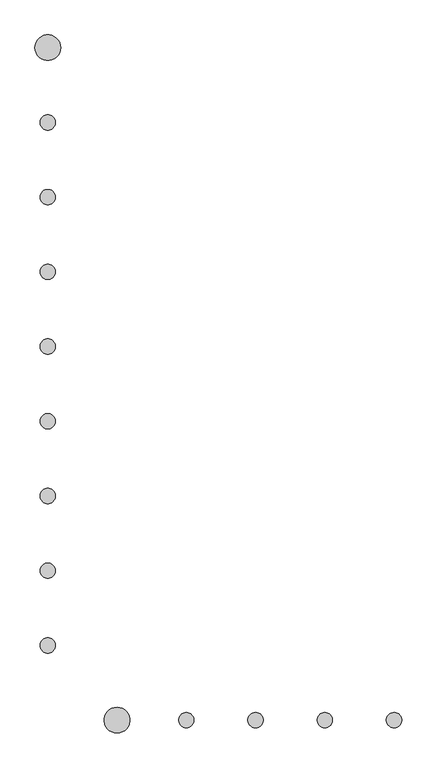
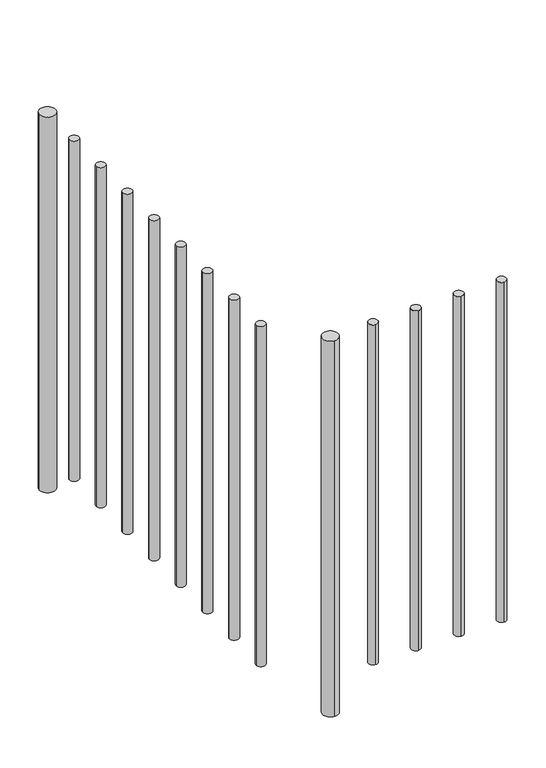
"""IFC4 building model written with IfcOpenShell, lengths in millimetres: railing geometry."""

import ifcopenshell
import ifcopenshell.guid

model = None  # the IFC model being written
_history = None  # IfcOwnerHistory: only IFC2X3 demands one
_inside = {}  # id of a spatial element -> (the spatial element, [elements in it])
_under = {}  # id of a project, library or spatial element -> (it, [spatial elements below it])
_declared = {}  # id of a project -> (the project, [libraries it declares])
_typed = {}  # id of a type object -> (the type object, [elements of that type])
_made_of = {}  # id of a material, layer set ... -> (it, [elements and type objects made of it])


def new_model(schema):
    """Start an empty IFC model of exactly this schema.

    Asked for "IFC4X3", IfcOpenShell would pick the latest addendum, in which some entities
    have other attributes; the version numbers below select the first issue.
    IFC2X3 requires an IfcOwnerHistory on every rooted entity: one is made here for all.
    """
    global model, _history
    if schema == "IFC4X3":
        model = ifcopenshell.file(schema_version=(4, 3, 0, 0))
    else:
        model = ifcopenshell.file(schema=schema)
    _inside.clear()
    _under.clear()
    _declared.clear()
    _typed.clear()
    _made_of.clear()
    _history = None
    if model.schema == "IFC2X3":
        org = make("IfcOrganization", Name="unknown")
        user = make(
            "IfcPersonAndOrganization",
            ThePerson=make("IfcPerson", FamilyName="unknown"),
            TheOrganization=org,
        )
        app = make(
            "IfcApplication",
            ApplicationDeveloper=org,
            Version="unknown",
            ApplicationFullName="unknown",
            ApplicationIdentifier="unknown",
        )
        _history = make(
            "IfcOwnerHistory",
            OwningUser=user,
            OwningApplication=app,
            ChangeAction="ADDED",
            CreationDate=0,
        )
    return model


def make(cls, **values):
    """One entity of the class cls with the attributes given. An attribute that is None is left unset."""
    return model.create_entity(
        cls, **{name: value for name, value in values.items() if value is not None}
    )


def rooted(cls, **values):
    """An entity with a GlobalId (a new one), such as an element, a storey or a relation."""
    return make(cls, GlobalId=ifcopenshell.guid.new(), OwnerHistory=_history, **values)


def si_unit(unit_type, name, prefix=None):
    """IfcSIUnit, for example si_unit("LENGTHUNIT", "METRE", prefix="MILLI")."""
    return make("IfcSIUnit", UnitType=unit_type, Prefix=prefix, Name=name)


def assignment(units):
    """IfcUnitAssignment: the units of a project."""
    return None if units is None else make("IfcUnitAssignment", Units=units)


def point(xyz):
    """IfcCartesianPoint."""
    return None if xyz is None else make("IfcCartesianPoint", Coordinates=xyz)


def direction(xyz):
    """IfcDirection."""
    return None if xyz is None else make("IfcDirection", DirectionRatios=xyz)


def frame(location, z_axis=None, x_axis=None):
    """IfcAxis2Placement3D, a coordinate frame: its origin and axes. An axis left out is left unset."""
    return make(
        "IfcAxis2Placement3D",
        Location=point(location),
        Axis=direction(z_axis),
        RefDirection=direction(x_axis),
    )


def frame_2d(location, x_axis=None):
    """IfcAxis2Placement2D, a coordinate frame in the plane: its origin and x axis."""
    return make(
        "IfcAxis2Placement2D", Location=point(location), RefDirection=direction(x_axis)
    )


def origin():
    """The frame at (0, 0, 0) with its axes left unset."""
    return frame((0.0, 0.0, 0.0))


def place(relative_to, where):
    """IfcLocalPlacement: puts the frame where relative to a parent placement (None: the world)."""
    return make(
        "IfcLocalPlacement", PlacementRelTo=relative_to, RelativePlacement=where
    )


def context(
    kind, dimensions, precision=None, world=None, true_north=None, identifier=None
):
    """IfcGeometricRepresentationContext, for example the 3D "Model" context."""
    return make(
        "IfcGeometricRepresentationContext",
        ContextIdentifier=identifier,
        ContextType=kind,
        CoordinateSpaceDimension=dimensions,
        Precision=precision,
        WorldCoordinateSystem=world,
        TrueNorth=true_north,
    )


def project(units=None, contexts=None):
    """IfcProject with its units and contexts."""
    return rooted(
        "IfcProject",
        Name="project",
        RepresentationContexts=contexts,
        UnitsInContext=assignment(units),
    )


def spatial(cls, under=None, at=None, **own):
    """A site, building, storey or space (cls), placed at a placement, below another one or the project."""
    s = rooted(cls, ObjectPlacement=at, **own)
    if under is not None:
        _under.setdefault(under.id(), (under, []))[1].append(s)
    return s


def circle_curve(where, radius):
    """IfcCircle in the frame where."""
    return make("IfcCircle", Position=where, Radius=radius)


def trimmed(basis, trim1, trim2, sense, master):
    """IfcTrimmedCurve: the piece of a basis curve between two trims."""
    return make(
        "IfcTrimmedCurve",
        BasisCurve=basis,
        Trim1=trim1,
        Trim2=trim2,
        SenseAgreement=sense,
        MasterRepresentation=master,
    )


def segment(curve, same_sense, transition):
    """IfcCompositeCurveSegment."""
    return make(
        "IfcCompositeCurveSegment",
        Transition=transition,
        SameSense=same_sense,
        ParentCurve=curve,
    )


def composite_curve(segments, self_intersect=None):
    """IfcCompositeCurve: segments joined end to end."""
    return make("IfcCompositeCurve", Segments=segments, SelfIntersect=self_intersect)


def outline(outer, holes=None, kind="AREA"):
    """IfcArbitraryClosedProfileDef: a profile drawn as a closed curve; with holes, ...WithVoids."""
    if holes is None:
        return make("IfcArbitraryClosedProfileDef", ProfileType=kind, OuterCurve=outer)
    return make(
        "IfcArbitraryProfileDefWithVoids",
        ProfileType=kind,
        OuterCurve=outer,
        InnerCurves=holes,
    )


def extrude(swept, where, along, depth):
    """IfcExtrudedAreaSolid: the profile swept, set in the frame where, extruded along a direction by depth."""
    return make(
        "IfcExtrudedAreaSolid",
        SweptArea=swept,
        Position=where,
        ExtrudedDirection=direction(along),
        Depth=depth,
    )


def shape(context_of_items, identifier, shape_type, items):
    """IfcShapeRepresentation: the items that make up one representation, for example the "Body"."""
    return make(
        "IfcShapeRepresentation",
        ContextOfItems=context_of_items,
        RepresentationIdentifier=identifier,
        RepresentationType=shape_type,
        Items=items,
    )


def source(mapping_origin, context_of_items, identifier, shape_type, items):
    """IfcRepresentationMap: a shape defined once, which mapped items show again and again."""
    return make(
        "IfcRepresentationMap",
        MappingOrigin=mapping_origin,
        MappedRepresentation=shape(context_of_items, identifier, shape_type, items),
    )


def transform(
    local_origin,
    x_axis=None,
    y_axis=None,
    z_axis=None,
    scale=None,
    scale2=None,
    scale3=None,
    uniform=True,
):
    """IfcCartesianTransformationOperator3D, or its non-uniform kind. x_axis, y_axis, z_axis: its Axis1, 2, 3."""
    if uniform:
        return make(
            "IfcCartesianTransformationOperator3D",
            Axis1=direction(x_axis),
            Axis2=direction(y_axis),
            LocalOrigin=point(local_origin),
            Scale=scale,
            Axis3=direction(z_axis),
        )
    return make(
        "IfcCartesianTransformationOperator3DnonUniform",
        Axis1=direction(x_axis),
        Axis2=direction(y_axis),
        LocalOrigin=point(local_origin),
        Scale=scale,
        Axis3=direction(z_axis),
        Scale2=scale2,
        Scale3=scale3,
    )


def mapped(mapping_source, mapping_target):
    """IfcMappedItem: shows the shape of a source again, moved by a transform."""
    return make(
        "IfcMappedItem", MappingSource=mapping_source, MappingTarget=mapping_target
    )


def made_of(thing, what):
    """Note that an element or type object is made of a material, layer set ...; save() writes the relation."""
    if what is not None:
        _made_of.setdefault(what.id(), (what, []))[1].append(thing)
    return thing


def element(
    cls,
    number,
    at=None,
    inside=None,
    cuts=None,
    type_object=None,
    material=None,
    context=None,
    identifier="Body",
    shape_type=None,
    held_by="IfcProductDefinitionShape",
    body=None,
    shapes=None,
    **own,
):
    """One element of the class cls, such as IfcWall. Its Tag is "e" and its number.

    at: its placement. inside: the storey or other place that contains it. cuts: it is an
    opening in that element (IfcRelVoidsElement). A single representation is given by context,
    identifier, shape_type and body (its items); several are given by shapes. held_by: the class
    of the entity that holds the representations. save() writes the other relations.
    """
    e = rooted(cls, Tag="e%d" % number, ObjectPlacement=at, **own)
    if body is not None:
        shapes = [shape(context, identifier, shape_type, body)]
    if shapes is not None:
        e.Representation = make(held_by, Representations=shapes)
    if inside is not None:
        _inside.setdefault(inside.id(), (inside, []))[1].append(e)
    if cuts is not None:
        rooted(
            "IfcRelVoidsElement", RelatingBuildingElement=cuts, RelatedOpeningElement=e
        )
    if type_object is not None:
        _typed.setdefault(type_object.id(), (type_object, []))[1].append(e)
    return made_of(e, material)


def aggregate(whole, parts):
    """IfcRelAggregates: a whole, such as a stair, and the parts it consists of."""
    return rooted("IfcRelAggregates", RelatingObject=whole, RelatedObjects=parts)


def save(model, path):
    """Write the relations noted so far, then the file.

    IfcRelAggregates (storeys below a building ...), IfcRelContainedInSpatialStructure (elements
    in a storey), IfcRelDefinesByType, IfcRelAssociatesMaterial and IfcRelDeclares: one each for
    every whole, place, type object, material and project.
    """
    for whole, parts in _under.values():
        aggregate(whole, parts)
    for where, things in _inside.values():
        rooted(
            "IfcRelContainedInSpatialStructure",
            RelatedElements=things,
            RelatingStructure=where,
        )
    for kind, things in _typed.values():
        rooted("IfcRelDefinesByType", RelatedObjects=things, RelatingType=kind)
    for what, things in _made_of.values():
        rooted("IfcRelAssociatesMaterial", RelatedObjects=things, RelatingMaterial=what)
    for by, libraries in _declared.values():
        rooted("IfcRelDeclares", RelatingContext=by, RelatedDefinitions=libraries)
    model.write(path)


def railing_35eac12f(model_context):
    return source(origin(), model_context, "Body", "SweptSolid", [
        extrude(outline(composite_curve([segment(trimmed(circle_curve(frame_2d((-2709.174449, -8163.7965465)), 12.5), [point((-2709.174449, -8176.2965465))], [point((-2709.174449, -8151.2965465))], False, "CARTESIAN"), True, "CONTINUOUS"), segment(trimmed(circle_curve(frame_2d((-2709.174449, -8163.7965465)), 12.5), [point((-2709.174449, -8151.2965465))], [point((-2709.174449, -8176.2965465))], False, "CARTESIAN"), True, "CONTINUOUS")], self_intersect=False)), frame((0.0, 0.0, 3500.0), z_axis=(0.0, 0.0, 1.0), x_axis=(1.0, 0.0, 0.0)), (0.0, 0.0, 1.0), 949.2),
        extrude(outline(composite_curve([segment(trimmed(circle_curve(frame_2d((-2822.314449, -8163.7965465)), 12.5), [point((-2822.314449, -8176.2965465))], [point((-2822.314449, -8151.2965465))], False, "CARTESIAN"), True, "CONTINUOUS"), segment(trimmed(circle_curve(frame_2d((-2822.314449, -8163.7965465)), 12.5), [point((-2822.314449, -8151.2965465))], [point((-2822.314449, -8176.2965465))], False, "CARTESIAN"), True, "CONTINUOUS")], self_intersect=False)), frame((0.0, 0.0, 3500.0), z_axis=(0.0, 0.0, 1.0), x_axis=(1.0, 0.0, 0.0)), (0.0, 0.0, 1.0), 949.2),
        extrude(outline(composite_curve([segment(trimmed(circle_curve(frame_2d((-2935.454449, -8163.7965465)), 12.5), [point((-2935.454449, -8176.2965465))], [point((-2935.454449, -8151.2965465))], False, "CARTESIAN"), True, "CONTINUOUS"), segment(trimmed(circle_curve(frame_2d((-2935.454449, -8163.7965465)), 12.5), [point((-2935.454449, -8151.2965465))], [point((-2935.454449, -8176.2965465))], False, "CARTESIAN"), True, "CONTINUOUS")], self_intersect=False)), frame((0.0, 0.0, 3500.0), z_axis=(0.0, 0.0, 1.0), x_axis=(1.0, 0.0, 0.0)), (0.0, 0.0, 1.0), 949.2),
        extrude(outline(composite_curve([segment(trimmed(circle_curve(frame_2d((-3048.594449, -8163.7965465)), 12.5), [point((-3048.594449, -8176.2965465))], [point((-3048.594449, -8151.2965465))], False, "CARTESIAN"), True, "CONTINUOUS"), segment(trimmed(circle_curve(frame_2d((-3048.594449, -8163.7965465)), 12.5), [point((-3048.594449, -8151.2965465))], [point((-3048.594449, -8176.2965465))], False, "CARTESIAN"), True, "CONTINUOUS")], self_intersect=False)), frame((0.0, 0.0, 3500.0), z_axis=(0.0, 0.0, 1.0), x_axis=(1.0, 0.0, 0.0)), (0.0, 0.0, 1.0), 949.2),
        extrude(outline(composite_curve([segment(trimmed(circle_curve(frame_2d((-3161.734449, -8163.7965465)), 21.0), [point((-3161.734449, -8184.7965465))], [point((-3161.734449, -8142.7965465))], False, "CARTESIAN"), True, "CONTINUOUS"), segment(trimmed(circle_curve(frame_2d((-3161.734449, -8163.7965465)), 21.0), [point((-3161.734449, -8142.7965465))], [point((-3161.734449, -8184.7965465))], False, "CARTESIAN"), True, "CONTINUOUS")], self_intersect=False)), frame((0.0, 0.0, 3400.0), z_axis=(0.0, 0.0, 1.0), x_axis=(1.0, 0.0, 0.0)), (0.0, 0.0, 1.0), 1049.2),
        extrude(outline(composite_curve([segment(trimmed(circle_curve(frame_2d((-3274.874449, -8041.7565465)), 12.5), [point((-3287.374449, -8041.7565465))], [point((-3262.374449, -8041.7565465))], False, "CARTESIAN"), True, "CONTINUOUS"), segment(trimmed(circle_curve(frame_2d((-3274.874449, -8041.7565465)), 12.5), [point((-3262.374449, -8041.7565465))], [point((-3287.374449, -8041.7565465))], False, "CARTESIAN"), True, "CONTINUOUS")], self_intersect=False)), frame((0.0, 0.0, 3500.0), z_axis=(0.0, 0.0, 1.0), x_axis=(1.0, 0.0, 0.0)), (0.0, 0.0, 1.0), 949.2),
        extrude(outline(composite_curve([segment(trimmed(circle_curve(frame_2d((-3274.874449, -7919.7165465)), 12.5), [point((-3287.374449, -7919.7165465))], [point((-3262.374449, -7919.7165465))], False, "CARTESIAN"), True, "CONTINUOUS"), segment(trimmed(circle_curve(frame_2d((-3274.874449, -7919.7165465)), 12.5), [point((-3262.374449, -7919.7165465))], [point((-3287.374449, -7919.7165465))], False, "CARTESIAN"), True, "CONTINUOUS")], self_intersect=False)), frame((0.0, 0.0, 3500.0), z_axis=(0.0, 0.0, 1.0), x_axis=(1.0, 0.0, 0.0)), (0.0, 0.0, 1.0), 949.2),
        extrude(outline(composite_curve([segment(trimmed(circle_curve(frame_2d((-3274.874449, -7797.6765465)), 12.5), [point((-3287.374449, -7797.6765465))], [point((-3262.374449, -7797.6765465))], False, "CARTESIAN"), True, "CONTINUOUS"), segment(trimmed(circle_curve(frame_2d((-3274.874449, -7797.6765465)), 12.5), [point((-3262.374449, -7797.6765465))], [point((-3287.374449, -7797.6765465))], False, "CARTESIAN"), True, "CONTINUOUS")], self_intersect=False)), frame((0.0, 0.0, 3500.0), z_axis=(0.0, 0.0, 1.0), x_axis=(1.0, 0.0, 0.0)), (0.0, 0.0, 1.0), 949.2),
        extrude(outline(composite_curve([segment(trimmed(circle_curve(frame_2d((-3274.874449, -7675.6365465)), 12.5), [point((-3287.374449, -7675.6365465))], [point((-3262.374449, -7675.6365465))], False, "CARTESIAN"), True, "CONTINUOUS"), segment(trimmed(circle_curve(frame_2d((-3274.874449, -7675.6365465)), 12.5), [point((-3262.374449, -7675.6365465))], [point((-3287.374449, -7675.6365465))], False, "CARTESIAN"), True, "CONTINUOUS")], self_intersect=False)), frame((0.0, 0.0, 3500.0), z_axis=(0.0, 0.0, 1.0), x_axis=(1.0, 0.0, 0.0)), (0.0, 0.0, 1.0), 949.2),
        extrude(outline(composite_curve([segment(trimmed(circle_curve(frame_2d((-3274.874449, -7553.5965465)), 12.5), [point((-3287.374449, -7553.5965465))], [point((-3262.374449, -7553.5965465))], False, "CARTESIAN"), True, "CONTINUOUS"), segment(trimmed(circle_curve(frame_2d((-3274.874449, -7553.5965465)), 12.5), [point((-3262.374449, -7553.5965465))], [point((-3287.374449, -7553.5965465))], False, "CARTESIAN"), True, "CONTINUOUS")], self_intersect=False)), frame((0.0, 0.0, 3500.0), z_axis=(0.0, 0.0, 1.0), x_axis=(1.0, 0.0, 0.0)), (0.0, 0.0, 1.0), 949.2),
        extrude(outline(composite_curve([segment(trimmed(circle_curve(frame_2d((-3274.874449, -7431.5565465)), 12.5), [point((-3287.374449, -7431.5565465))], [point((-3262.374449, -7431.5565465))], False, "CARTESIAN"), True, "CONTINUOUS"), segment(trimmed(circle_curve(frame_2d((-3274.874449, -7431.5565465)), 12.5), [point((-3262.374449, -7431.5565465))], [point((-3287.374449, -7431.5565465))], False, "CARTESIAN"), True, "CONTINUOUS")], self_intersect=False)), frame((0.0, 0.0, 3500.0), z_axis=(0.0, 0.0, 1.0), x_axis=(1.0, 0.0, 0.0)), (0.0, 0.0, 1.0), 949.2),
        extrude(outline(composite_curve([segment(trimmed(circle_curve(frame_2d((-3274.874449, -7309.5165465)), 12.5), [point((-3287.374449, -7309.5165465))], [point((-3262.374449, -7309.5165465))], False, "CARTESIAN"), True, "CONTINUOUS"), segment(trimmed(circle_curve(frame_2d((-3274.874449, -7309.5165465)), 12.5), [point((-3262.374449, -7309.5165465))], [point((-3287.374449, -7309.5165465))], False, "CARTESIAN"), True, "CONTINUOUS")], self_intersect=False)), frame((0.0, 0.0, 3500.0), z_axis=(0.0, 0.0, 1.0), x_axis=(1.0, 0.0, 0.0)), (0.0, 0.0, 1.0), 949.2),
        extrude(outline(composite_curve([segment(trimmed(circle_curve(frame_2d((-3274.874449, -7187.4765465)), 12.5), [point((-3287.374449, -7187.4765465))], [point((-3262.374449, -7187.4765465))], False, "CARTESIAN"), True, "CONTINUOUS"), segment(trimmed(circle_curve(frame_2d((-3274.874449, -7187.4765465)), 12.5), [point((-3262.374449, -7187.4765465))], [point((-3287.374449, -7187.4765465))], False, "CARTESIAN"), True, "CONTINUOUS")], self_intersect=False)), frame((0.0, 0.0, 3500.0), z_axis=(0.0, 0.0, 1.0), x_axis=(1.0, 0.0, 0.0)), (0.0, 0.0, 1.0), 949.2),
        extrude(outline(composite_curve([segment(trimmed(circle_curve(frame_2d((-3274.874449, -7065.4365465)), 21.0), [point((-3295.874449, -7065.4365465))], [point((-3253.874449, -7065.4365465))], False, "CARTESIAN"), True, "CONTINUOUS"), segment(trimmed(circle_curve(frame_2d((-3274.874449, -7065.4365465)), 21.0), [point((-3253.874449, -7065.4365465))], [point((-3295.874449, -7065.4365465))], False, "CARTESIAN"), True, "CONTINUOUS")], self_intersect=False)), frame((0.0, 0.0, 3400.0), z_axis=(0.0, 0.0, 1.0), x_axis=(1.0, 0.0, 0.0)), (0.0, 0.0, 1.0), 1049.2),
    ])


if __name__ == "__main__":
    model = new_model("IFC4")
    model_context = context("Model", 3, world=origin())
    ifc_project = project(units=[si_unit("LENGTHUNIT", "METRE", prefix="MILLI")], contexts=[model_context])
    site = spatial("IfcSite", under=ifc_project)
    building = spatial("IfcBuilding", under=site)
    placement = place(None, origin())
    railing_shape = railing_35eac12f(model_context)
    element("IfcRailing", 1, at=placement, inside=building, context=model_context, shape_type="MappedRepresentation", body=[
        mapped(railing_shape, transform((0.0, 0.0, 0.0), x_axis=(1.0, 0.0, 0.0), y_axis=(0.0, 1.0, 0.0), z_axis=(0.0, 0.0, 1.0))),
    ])
    save(model, "model.ifc")

# Revit data of these elements
# Project information
#   Project Issue Date = "Data de emissão"
#   Project Status = "Status do projeto"
#   Client Name = "Proprietário"
#   Project Address = "Insira aqui o endereço"
#   Project Name = "Nome do projeto"
#   Project Number = "0001"
# Element 1 (IfcRailing)
#   Materials on its faces: "Ferro - Pintura Esmalte"
# Materials
#   "Ferro - Pintura Esmalte": class "Pintura", colour RGB 255 255 255, transparency 0, Cost = 0
